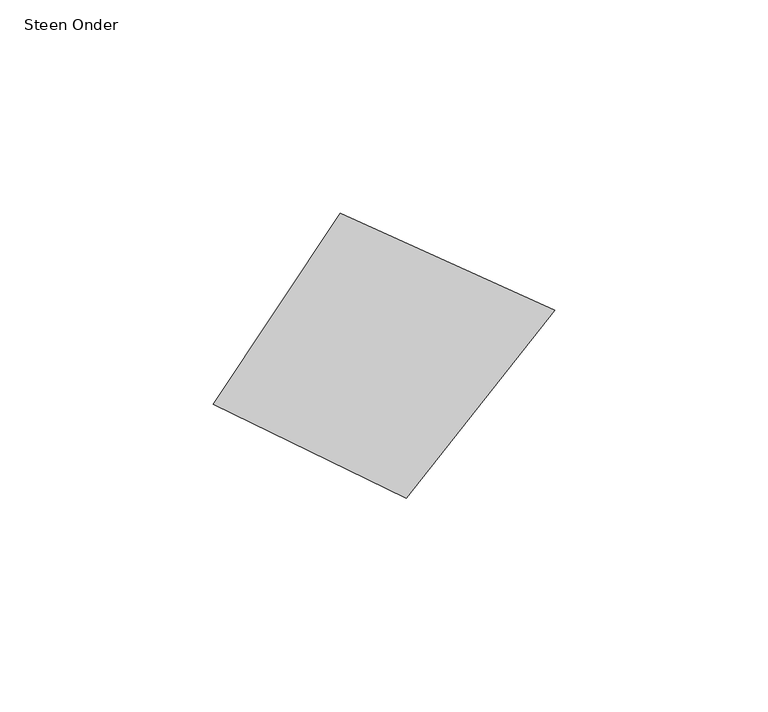
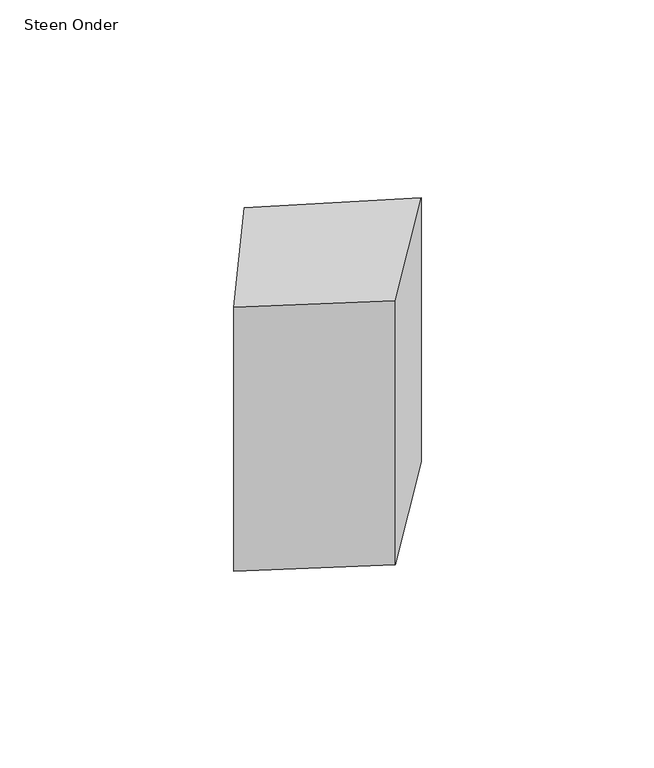
"""IFC4 building model written with IfcOpenShell, lengths in millimetres: proxy geometry, 00_GMA_steen_versie_4 : Steen Onder."""

from ifc_helpers import new_model, si_unit, frame, origin, place, context, project, spatial, polyline, outline, extrude, source, transform, mapped, element, save


def steen_onder_ca3ff13a(model_context):
    return source(origin(), model_context, "Body", "SweptSolid", [
        extrude(outline(polyline([(125.6273492, 54.1515578), (90.8788668, 10.0356349), (45.6534224, 32.0397224), (75.3550053, 76.8203564), (125.6273492, 54.1515578)])), frame((0.0, 0.0, -100.0), z_axis=(0.0, 0.0, 1.0), x_axis=(1.0, 0.0, 0.0)), (0.0, 0.0, 1.0), 100.0),
    ])


if __name__ == "__main__":
    model = new_model("IFC4")
    model_context = context("Model", 3, world=origin())
    ifc_project = project(units=[si_unit("LENGTHUNIT", "METRE", prefix="MILLI")], contexts=[model_context])
    site = spatial("IfcSite", under=ifc_project)
    building = spatial("IfcBuilding", under=site)
    placement = place(None, origin())
    steen_onder_shape = steen_onder_ca3ff13a(model_context)
    element("IfcBuildingElementProxy", 1, Name="00_GMA_steen_versie_4 : Steen Onder", ObjectType="00_GMA_steen_versie_4 : Steen Onder", at=placement, inside=building, context=model_context, shape_type="MappedRepresentation", body=[
        mapped(steen_onder_shape, transform((0.0, 0.0, 0.0), x_axis=(1.0, 0.0, 0.0), y_axis=(0.0, 1.0, 0.0), z_axis=(0.0, 0.0, 1.0))),
    ])
    save(model, "model.ifc")

# Revit data of these elements
# Type "00_GMA_steen_versie_4 : Steen Onder"
#   StootVoegHalfBoven [instance default] = 5 mm
#   StootVoegHalf [instance default] = 5 mm
#   StootVoegBreedteOnder = 10 mm
#   StootVoegBreedteBoven = 10 mm
#   Steendikte = 100 mm
#   LintVoegOnderHalf = 0 mm
#   LintVoegOnder = 0 mm
#   LintVoegBovenHalf = 5 mm
#   LintVoegBoven = 10 mm
#   materiaal = none
#   MateriaalVoeg = none
#   Default Elevation = 0
